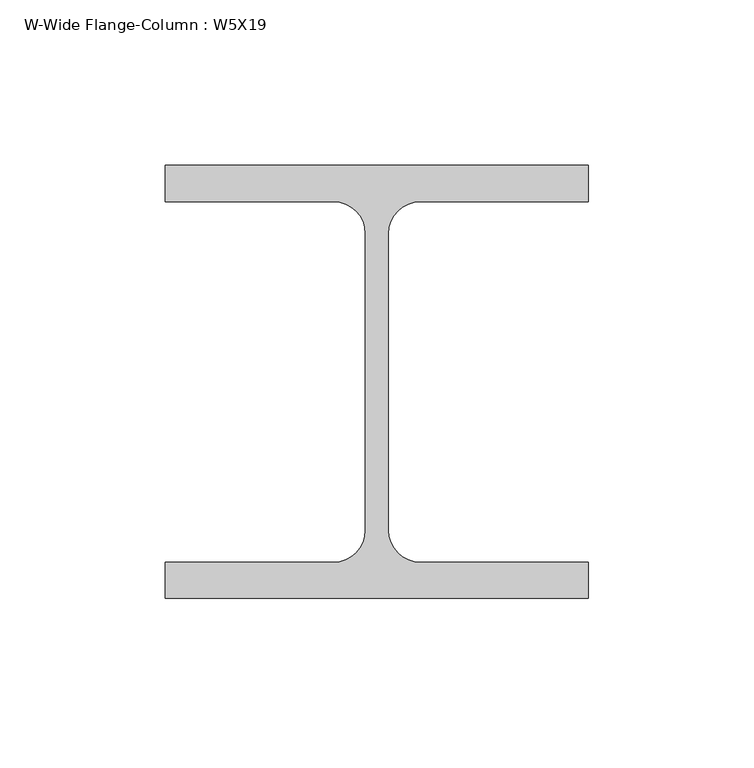
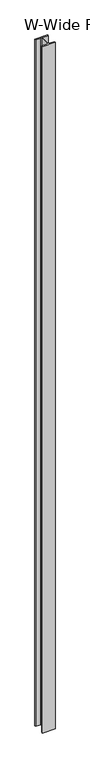
"""IFC4 building model written with IfcOpenShell, lengths in millimetres: column geometry, W-Wide Flange-Column : W5X19."""

import ifcopenshell
import ifcopenshell.guid

model = None  # the IFC model being written
_history = None  # IfcOwnerHistory: only IFC2X3 demands one
_inside = {}  # id of a spatial element -> (the spatial element, [elements in it])
_under = {}  # id of a project, library or spatial element -> (it, [spatial elements below it])
_declared = {}  # id of a project -> (the project, [libraries it declares])
_typed = {}  # id of a type object -> (the type object, [elements of that type])
_made_of = {}  # id of a material, layer set ... -> (it, [elements and type objects made of it])


def new_model(schema):
    """Start an empty IFC model of exactly this schema.

    Asked for "IFC4X3", IfcOpenShell would pick the latest addendum, in which some entities
    have other attributes; the version numbers below select the first issue.
    IFC2X3 requires an IfcOwnerHistory on every rooted entity: one is made here for all.
    """
    global model, _history
    if schema == "IFC4X3":
        model = ifcopenshell.file(schema_version=(4, 3, 0, 0))
    else:
        model = ifcopenshell.file(schema=schema)
    _inside.clear()
    _under.clear()
    _declared.clear()
    _typed.clear()
    _made_of.clear()
    _history = None
    if model.schema == "IFC2X3":
        org = make("IfcOrganization", Name="unknown")
        user = make(
            "IfcPersonAndOrganization",
            ThePerson=make("IfcPerson", FamilyName="unknown"),
            TheOrganization=org,
        )
        app = make(
            "IfcApplication",
            ApplicationDeveloper=org,
            Version="unknown",
            ApplicationFullName="unknown",
            ApplicationIdentifier="unknown",
        )
        _history = make(
            "IfcOwnerHistory",
            OwningUser=user,
            OwningApplication=app,
            ChangeAction="ADDED",
            CreationDate=0,
        )
    return model


def make(cls, **values):
    """One entity of the class cls with the attributes given. An attribute that is None is left unset."""
    return model.create_entity(
        cls, **{name: value for name, value in values.items() if value is not None}
    )


def rooted(cls, **values):
    """An entity with a GlobalId (a new one), such as an element, a storey or a relation."""
    return make(cls, GlobalId=ifcopenshell.guid.new(), OwnerHistory=_history, **values)


def si_unit(unit_type, name, prefix=None):
    """IfcSIUnit, for example si_unit("LENGTHUNIT", "METRE", prefix="MILLI")."""
    return make("IfcSIUnit", UnitType=unit_type, Prefix=prefix, Name=name)


def assignment(units):
    """IfcUnitAssignment: the units of a project."""
    return None if units is None else make("IfcUnitAssignment", Units=units)


def point(xyz):
    """IfcCartesianPoint."""
    return None if xyz is None else make("IfcCartesianPoint", Coordinates=xyz)


def direction(xyz):
    """IfcDirection."""
    return None if xyz is None else make("IfcDirection", DirectionRatios=xyz)


def frame(location, z_axis=None, x_axis=None):
    """IfcAxis2Placement3D, a coordinate frame: its origin and axes. An axis left out is left unset."""
    return make(
        "IfcAxis2Placement3D",
        Location=point(location),
        Axis=direction(z_axis),
        RefDirection=direction(x_axis),
    )


def frame_2d(location, x_axis=None):
    """IfcAxis2Placement2D, a coordinate frame in the plane: its origin and x axis."""
    return make(
        "IfcAxis2Placement2D", Location=point(location), RefDirection=direction(x_axis)
    )


def origin():
    """The frame at (0, 0, 0) with its axes left unset."""
    return frame((0.0, 0.0, 0.0))


def origin_with_axes():
    """The frame at (0, 0, 0) with the z axis (0, 0, 1) and the x axis (1, 0, 0) written out."""
    return frame((0.0, 0.0, 0.0), z_axis=(0.0, 0.0, 1.0), x_axis=(1.0, 0.0, 0.0))


def place(relative_to, where):
    """IfcLocalPlacement: puts the frame where relative to a parent placement (None: the world)."""
    return make(
        "IfcLocalPlacement", PlacementRelTo=relative_to, RelativePlacement=where
    )


def context(
    kind, dimensions, precision=None, world=None, true_north=None, identifier=None
):
    """IfcGeometricRepresentationContext, for example the 3D "Model" context."""
    return make(
        "IfcGeometricRepresentationContext",
        ContextIdentifier=identifier,
        ContextType=kind,
        CoordinateSpaceDimension=dimensions,
        Precision=precision,
        WorldCoordinateSystem=world,
        TrueNorth=true_north,
    )


def project(units=None, contexts=None):
    """IfcProject with its units and contexts."""
    return rooted(
        "IfcProject",
        Name="project",
        RepresentationContexts=contexts,
        UnitsInContext=assignment(units),
    )


def spatial(cls, under=None, at=None, **own):
    """A site, building, storey or space (cls), placed at a placement, below another one or the project."""
    s = rooted(cls, ObjectPlacement=at, **own)
    if under is not None:
        _under.setdefault(under.id(), (under, []))[1].append(s)
    return s


def polyline(points):
    """IfcPolyline through the points."""
    return make("IfcPolyline", Points=[point(p) for p in points])


def circle_curve(where, radius):
    """IfcCircle in the frame where."""
    return make("IfcCircle", Position=where, Radius=radius)


def trimmed(basis, trim1, trim2, sense, master):
    """IfcTrimmedCurve: the piece of a basis curve between two trims."""
    return make(
        "IfcTrimmedCurve",
        BasisCurve=basis,
        Trim1=trim1,
        Trim2=trim2,
        SenseAgreement=sense,
        MasterRepresentation=master,
    )


def segment(curve, same_sense, transition):
    """IfcCompositeCurveSegment."""
    return make(
        "IfcCompositeCurveSegment",
        Transition=transition,
        SameSense=same_sense,
        ParentCurve=curve,
    )


def composite_curve(segments, self_intersect=None):
    """IfcCompositeCurve: segments joined end to end."""
    return make("IfcCompositeCurve", Segments=segments, SelfIntersect=self_intersect)


def outline(outer, holes=None, kind="AREA"):
    """IfcArbitraryClosedProfileDef: a profile drawn as a closed curve; with holes, ...WithVoids."""
    if holes is None:
        return make("IfcArbitraryClosedProfileDef", ProfileType=kind, OuterCurve=outer)
    return make(
        "IfcArbitraryProfileDefWithVoids",
        ProfileType=kind,
        OuterCurve=outer,
        InnerCurves=holes,
    )


def extrude(swept, where, along, depth):
    """IfcExtrudedAreaSolid: the profile swept, set in the frame where, extruded along a direction by depth."""
    return make(
        "IfcExtrudedAreaSolid",
        SweptArea=swept,
        Position=where,
        ExtrudedDirection=direction(along),
        Depth=depth,
    )


def shape(context_of_items, identifier, shape_type, items):
    """IfcShapeRepresentation: the items that make up one representation, for example the "Body"."""
    return make(
        "IfcShapeRepresentation",
        ContextOfItems=context_of_items,
        RepresentationIdentifier=identifier,
        RepresentationType=shape_type,
        Items=items,
    )


def source(mapping_origin, context_of_items, identifier, shape_type, items):
    """IfcRepresentationMap: a shape defined once, which mapped items show again and again."""
    return make(
        "IfcRepresentationMap",
        MappingOrigin=mapping_origin,
        MappedRepresentation=shape(context_of_items, identifier, shape_type, items),
    )


def transform(
    local_origin,
    x_axis=None,
    y_axis=None,
    z_axis=None,
    scale=None,
    scale2=None,
    scale3=None,
    uniform=True,
):
    """IfcCartesianTransformationOperator3D, or its non-uniform kind. x_axis, y_axis, z_axis: its Axis1, 2, 3."""
    if uniform:
        return make(
            "IfcCartesianTransformationOperator3D",
            Axis1=direction(x_axis),
            Axis2=direction(y_axis),
            LocalOrigin=point(local_origin),
            Scale=scale,
            Axis3=direction(z_axis),
        )
    return make(
        "IfcCartesianTransformationOperator3DnonUniform",
        Axis1=direction(x_axis),
        Axis2=direction(y_axis),
        LocalOrigin=point(local_origin),
        Scale=scale,
        Axis3=direction(z_axis),
        Scale2=scale2,
        Scale3=scale3,
    )


def mapped(mapping_source, mapping_target):
    """IfcMappedItem: shows the shape of a source again, moved by a transform."""
    return make(
        "IfcMappedItem", MappingSource=mapping_source, MappingTarget=mapping_target
    )


def made_of(thing, what):
    """Note that an element or type object is made of a material, layer set ...; save() writes the relation."""
    if what is not None:
        _made_of.setdefault(what.id(), (what, []))[1].append(thing)
    return thing


def element(
    cls,
    number,
    at=None,
    inside=None,
    cuts=None,
    type_object=None,
    material=None,
    context=None,
    identifier="Body",
    shape_type=None,
    held_by="IfcProductDefinitionShape",
    body=None,
    shapes=None,
    **own,
):
    """One element of the class cls, such as IfcWall. Its Tag is "e" and its number.

    at: its placement. inside: the storey or other place that contains it. cuts: it is an
    opening in that element (IfcRelVoidsElement). A single representation is given by context,
    identifier, shape_type and body (its items); several are given by shapes. held_by: the class
    of the entity that holds the representations. save() writes the other relations.
    """
    e = rooted(cls, Tag="e%d" % number, ObjectPlacement=at, **own)
    if body is not None:
        shapes = [shape(context, identifier, shape_type, body)]
    if shapes is not None:
        e.Representation = make(held_by, Representations=shapes)
    if inside is not None:
        _inside.setdefault(inside.id(), (inside, []))[1].append(e)
    if cuts is not None:
        rooted(
            "IfcRelVoidsElement", RelatingBuildingElement=cuts, RelatedOpeningElement=e
        )
    if type_object is not None:
        _typed.setdefault(type_object.id(), (type_object, []))[1].append(e)
    return made_of(e, material)


def aggregate(whole, parts):
    """IfcRelAggregates: a whole, such as a stair, and the parts it consists of."""
    return rooted("IfcRelAggregates", RelatingObject=whole, RelatedObjects=parts)


def save(model, path):
    """Write the relations noted so far, then the file.

    IfcRelAggregates (storeys below a building ...), IfcRelContainedInSpatialStructure (elements
    in a storey), IfcRelDefinesByType, IfcRelAssociatesMaterial and IfcRelDeclares: one each for
    every whole, place, type object, material and project.
    """
    for whole, parts in _under.values():
        aggregate(whole, parts)
    for where, things in _inside.values():
        rooted(
            "IfcRelContainedInSpatialStructure",
            RelatedElements=things,
            RelatingStructure=where,
        )
    for kind, things in _typed.values():
        rooted("IfcRelDefinesByType", RelatedObjects=things, RelatingType=kind)
    for what, things in _made_of.values():
        rooted("IfcRelAssociatesMaterial", RelatedObjects=things, RelatingMaterial=what)
    for by, libraries in _declared.values():
        rooted("IfcRelDeclares", RelatingContext=by, RelatedDefinitions=libraries)
    model.write(path)


def w_wide_flange_column_w5x19_9bf40364(model_context):
    return source(origin(), model_context, "Body", "SweptSolid", [
        extrude(outline(composite_curve([segment(polyline([(63.881, 65.405), (63.881, 54.483), (13.1445, 54.483)]), True, "CONTINUOUS"), segment(trimmed(circle_curve(frame_2d((13.1445, 44.7675)), 9.7155), [point((13.1445, 54.483))], [point((3.429, 44.7675))], True, "CARTESIAN"), True, "CONTINUOUS"), segment(polyline([(3.429, 44.7675), (3.429, -44.7675)]), True, "CONTINUOUS"), segment(trimmed(circle_curve(frame_2d((13.1445, -44.7675)), 9.7155), [point((3.429, -44.7675))], [point((13.1445, -54.483))], True, "CARTESIAN"), True, "CONTINUOUS"), segment(polyline([(13.1445, -54.483), (63.881, -54.483), (63.881, -65.405), (-63.881, -65.405), (-63.881, -54.483), (-13.1445, -54.483)]), True, "CONTINUOUS"), segment(trimmed(circle_curve(frame_2d((-13.1445, -44.7675)), 9.7155), [point((-13.1445, -54.483))], [point((-3.429, -44.7675))], True, "CARTESIAN"), True, "CONTINUOUS"), segment(polyline([(-3.429, -44.7675), (-3.429, 44.7675)]), True, "CONTINUOUS"), segment(trimmed(circle_curve(frame_2d((-13.1445, 44.7675)), 9.7155), [point((-3.429, 44.7675))], [point((-13.1445, 54.483))], True, "CARTESIAN"), True, "CONTINUOUS"), segment(polyline([(-13.1445, 54.483), (-63.881, 54.483), (-63.881, 65.405), (63.881, 65.405)]), True, "CONTINUOUS")], self_intersect=False)), origin_with_axes(), (0.0, 0.0, 1.0), 7315.2),
    ])


if __name__ == "__main__":
    model = new_model("IFC4")
    model_context = context("Model", 3, world=origin())
    ifc_project = project(units=[si_unit("LENGTHUNIT", "METRE", prefix="MILLI")], contexts=[model_context])
    site = spatial("IfcSite", under=ifc_project)
    building = spatial("IfcBuilding", under=site)
    placement = place(None, origin())
    w_wide_flange_column_w5x19_shape = w_wide_flange_column_w5x19_9bf40364(model_context)
    element("IfcColumn", 1, ObjectType="W-Wide Flange-Column : W5X19", at=placement, inside=building, context=model_context, shape_type="MappedRepresentation", body=[
        mapped(w_wide_flange_column_w5x19_shape, transform((0.0, 0.0, 0.0), x_axis=(1.0, 0.0, 0.0), y_axis=(0.0, 1.0, 0.0), z_axis=(0.0, 0.0, 1.0))),
    ])
    save(model, "model.ifc")

# Revit data of these elements
# Type "W-Wide Flange-Column : W5X19"
#   Assembly Code = "B10"
#   W = 19
#   bf = 127.762 mm
#   d = 130.81 mm
#   k = 20.638 mm
#   kr = 9.716 mm
#   tf = 10.922 mm
#   tw = 6.858 mm
#   A = 0.00358709 m²
#   Structural Material [instance default] = Metal - Steel - ASTM A992
# Element 1 (IfcColumn, "W-Wide Flange-Column : W5X19")
#   Materials on its faces: "Metal - Steel - ASTM A992"
# Materials
#   "Metal - Steel - ASTM A992": class "Metal", colour RGB 10 10 10, transparency 0
